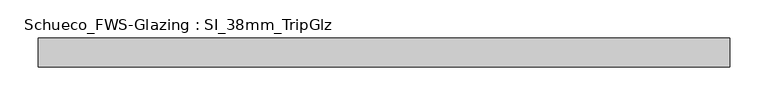
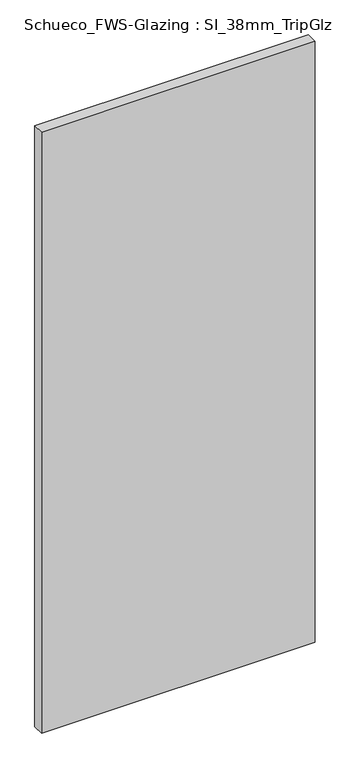
"""IFC4 building model written with IfcOpenShell, lengths in millimetres: plate geometry, Schueco_FWS-Glazing : SI_38mm_TripGlz."""

from ifc_helpers import new_model, si_unit, origin, origin_with_axes, place, context, project, spatial, polyline, outline, extrude, source, transform, mapped, element, save


def schueco_fws_glazing_si_38mm_tripglz_c3793eb7(model_context):
    return source(origin(), model_context, "Body", "SweptSolid", [
        extrude(outline(polyline([(454.0, -38.0), (-454.0, -38.0), (-454.0, 0.0), (454.0, 0.0), (454.0, -38.0)])), origin_with_axes(), (0.0, 0.0, 1.0), 2108.0),
    ])


if __name__ == "__main__":
    model = new_model("IFC4")
    model_context = context("Model", 3, world=origin())
    ifc_project = project(units=[si_unit("LENGTHUNIT", "METRE", prefix="MILLI")], contexts=[model_context])
    site = spatial("IfcSite", under=ifc_project)
    building = spatial("IfcBuilding", under=site)
    placement = place(None, origin())
    schueco_fws_glazing_si_38mm_tripglz_shape = schueco_fws_glazing_si_38mm_tripglz_c3793eb7(model_context)
    element("IfcPlate", 1, ObjectType="Schueco_FWS-Glazing : SI_38mm_TripGlz", at=placement, inside=building, context=model_context, shape_type="MappedRepresentation", body=[
        mapped(schueco_fws_glazing_si_38mm_tripglz_shape, transform((0.0, 0.0, 0.0), x_axis=(1.0, 0.0, 0.0), y_axis=(0.0, 1.0, 0.0), z_axis=(0.0, 0.0, 1.0))),
    ])
    save(model, "model.ifc")

# Revit data of these elements
# Type "Schueco_FWS-Glazing : SI_38mm_TripGlz"
#   Model = "Triple glazing 38mm"
#   Manufacturer = "Schueco International KG"
#   Analytic Construction = "<Keine Auswahl>"
#   Glazing thickness = 38 mm
#   FWS SI insert unit = yes
#   FWS HI insert unit = no
#   Glass = Glass
# Element 1 (IfcPlate, "Schueco_FWS-Glazing : SI_38mm_TripGlz")
#   Materials on its faces: "Glass"
# Materials
#   "Glass": class "Glass", colour RGB 128 128 255, transparency 0.75, Description = "Soda Lime Glass", Cost = 0
